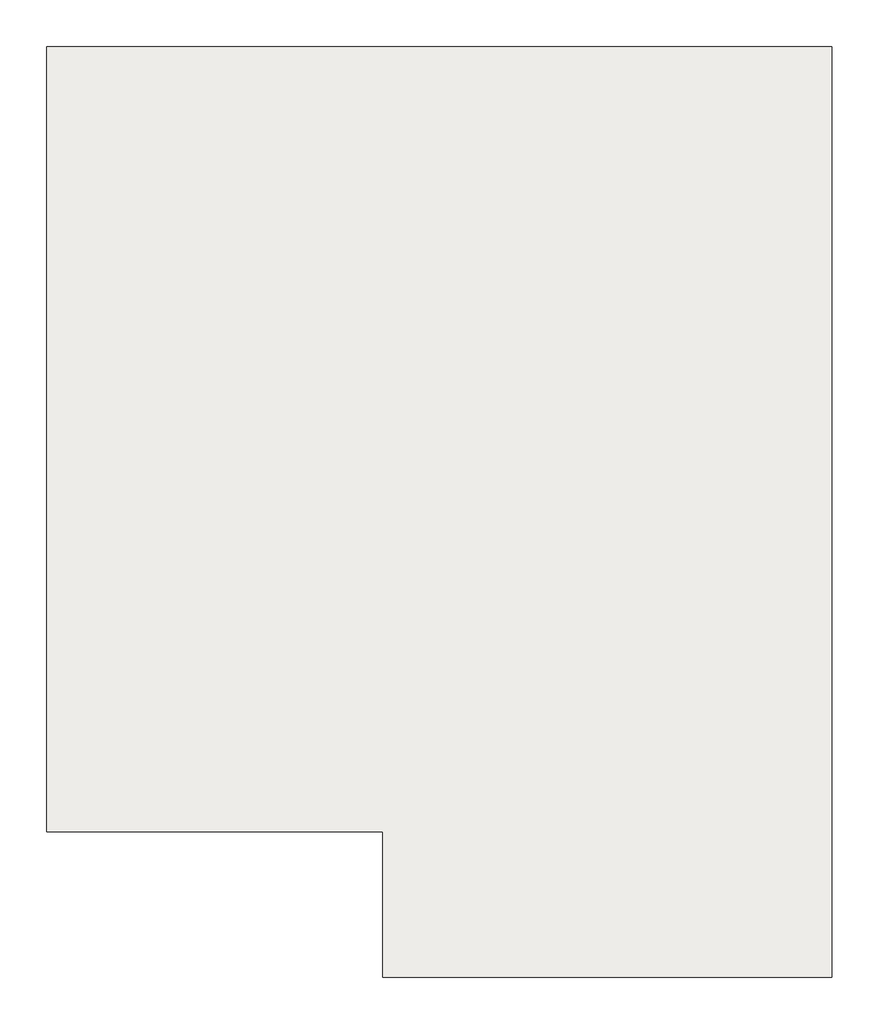
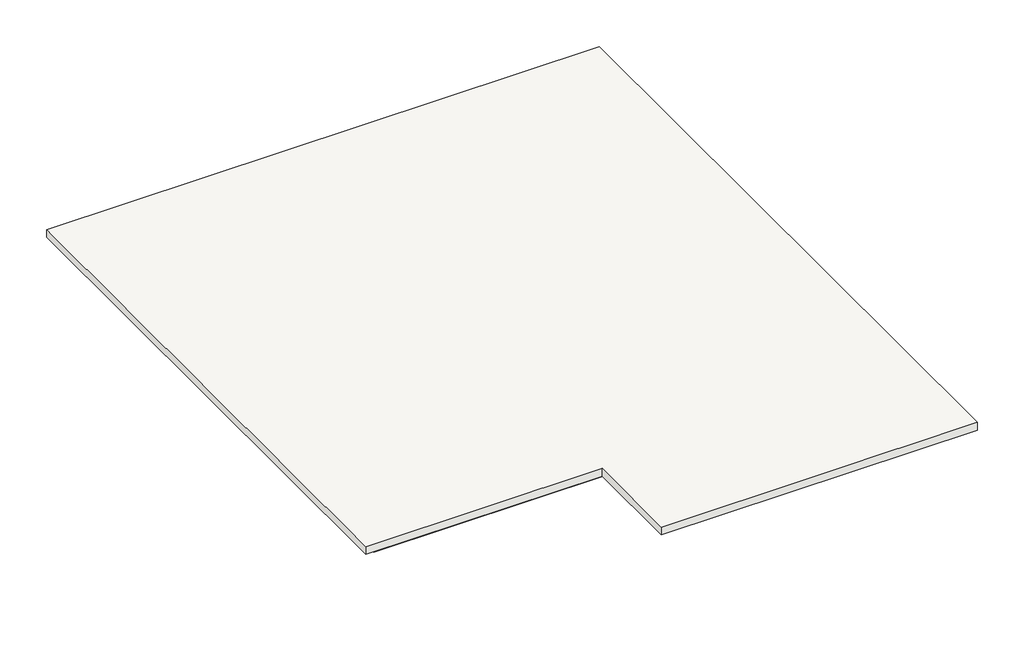
# One storey: 15 beams, 1 slab.
"""IFC4 building model written with IfcOpenShell, lengths in millimetres."""

from ifc_helpers import new_model, si_unit, frame, origin, place, context, project, spatial, polyline, outline, extrude, faceted_brep, element, save

model = new_model("IFC4")

# Units and contexts
model_context = context("Model", 3, world=origin())
ifc_project = project(units=[si_unit("LENGTHUNIT", "METRE", prefix="MILLI")], contexts=[model_context])

# Site, building, storey
site = spatial("IfcSite", under=ifc_project)
building = spatial("IfcBuilding", under=site)
storey = spatial("IfcBuildingStorey", under=building, Name="Çatı Katı", Elevation=100780.0)

# Beams
placement = place(None, origin())
element("IfcBeam", 1, ObjectType="M_Concrete-Rectangular Beam : 300 x 600mm", at=placement, inside=storey, context=model_context, shape_type="SweptSolid", body=[
    extrude(outline(polyline([(-8879.0485128, 8478.2904426), (-8879.0485128, 8778.2904426), (-5329.0485128, 8778.2904426), (-5329.0485128, 8478.2904426), (-8879.0485128, 8478.2904426)])), frame((0.0, 0.0, 100180.0), z_axis=(0.0, 0.0, 1.0), x_axis=(1.0, 0.0, 0.0)), (0.0, 0.0, 1.0), 400.0),
])
element("IfcBeam", 2, ObjectType="M_Concrete-Rectangular Beam : 300 x 600mm", at=placement, inside=storey, context=model_context, shape_type="SweptSolid", body=[
    extrude(outline(polyline([(-2679.0485128, 2578.2904426), (-2979.0485128, 2578.2904426), (-2979.0485128, 4628.2904426), (-2679.0485128, 4628.2904426), (-2679.0485128, 2578.2904426)])), frame((0.0, 0.0, 100180.0), z_axis=(0.0, 0.0, 1.0), x_axis=(1.0, 0.0, 0.0)), (0.0, 0.0, 1.0), 400.0),
])
element("IfcBeam", 3, ObjectType="M_Concrete-Rectangular Beam : 450 x 600mm", at=placement, inside=storey, context=model_context, shape_type="SweptSolid", body=[
    extrude(outline(polyline([(-8954.0485128, -3259.0095568), (-9404.0485128, -3259.0095568), (-9404.0485128, 1978.2904426), (-8954.0485128, 1978.2904426), (-8954.0485128, -3259.0095568)])), frame((0.0, 0.0, 100180.0), z_axis=(0.0, 0.0, 1.0), x_axis=(1.0, 0.0, 0.0)), (0.0, 0.0, 1.0), 400.0),
])
element("IfcBeam", 4, ObjectType="M_Concrete-Rectangular Beam : 450 x 600mm", at=placement, inside=storey, context=model_context, shape_type="SweptSolid", body=[
    extrude(outline(polyline([(-9404.0485128, 8315.590442), (-8954.0485128, 8315.590442), (-8954.0485128, 2578.2904426), (-9404.0485128, 2578.2904426), (-9404.0485128, 8315.590442)])), frame((0.0, 0.0, 100180.0), z_axis=(0.0, 0.0, 1.0), x_axis=(1.0, 0.0, 0.0)), (0.0, 0.0, 1.0), 400.0),
])
element("IfcBeam", 5, ObjectType="M_Concrete-Rectangular Beam : 450 x 600mm", at=placement, inside=storey, context=model_context, shape_type="SweptSolid", body=[
    extrude(outline(polyline([(-14716.3485122, 2053.2904426), (-14716.3485122, 2503.2904426), (-9404.0485128, 2503.2904426), (-9404.0485128, 2053.2904426), (-14716.3485122, 2053.2904426)])), frame((0.0, 0.0, 100180.0), z_axis=(0.0, 0.0, 1.0), x_axis=(1.0, 0.0, 0.0)), (0.0, 0.0, 1.0), 400.0),
])
element("IfcBeam", 6, ObjectType="M_Concrete-Rectangular Beam : 450 x 600mm", at=placement, inside=storey, context=model_context, shape_type="SweptSolid", body=[
    extrude(outline(polyline([(-3141.7485135, 2503.2904426), (-3141.7485135, 2053.2904426), (-8954.0485128, 2053.2904426), (-8954.0485128, 2503.2904426), (-3141.7485135, 2503.2904426)])), frame((0.0, 0.0, 100180.0), z_axis=(0.0, 0.0, 1.0), x_axis=(1.0, 0.0, 0.0)), (0.0, 0.0, 1.0), 400.0),
])
element("IfcBeam", 7, ObjectType="M_Concrete-Rectangular Beam : 450 x 600mm", at=placement, inside=storey, context=model_context, shape_type="SweptSolid", body=[
    extrude(outline(polyline([(-9491.7485135, 8803.2904426), (-9491.7485135, 8353.2904426), (-14729.0485128, 8353.2904426), (-14729.0485128, 8778.2904426), (-15179.0485128, 8778.2904426), (-15179.0485128, 8353.2904426), (-15204.0485128, 8353.2904426), (-15204.0485128, 8803.2904426), (-9491.7485135, 8803.2904426)])), frame((0.0, 0.0, 100180.0), z_axis=(0.0, 0.0, 1.0), x_axis=(1.0, 0.0, 0.0)), (0.0, 0.0, 1.0), 400.0),
])
element("IfcBeam", 8, ObjectType="M_Concrete-Rectangular Beam : 450 x 600mm", at=placement, inside=storey, context=model_context, shape_type="Brep", body=[
    faceted_brep([(-2654.0485128, 1965.590442, 100180.0), (-3104.0485128, 1965.590442, 100180.0), (-3104.0485128, 1965.590442, 100580.0), (-2654.0485128, 1965.590442, 100580.0), (-2654.0485128, -3746.7095574, 100180.0), (-2654.0485128, -3746.7095574, 100580.0), (-2679.0485128, -3746.7095574, 100180.0), (-3104.0485128, -3746.7095574, 100180.0), (-3104.0485128, -3721.7095574, 100180.0), (-2679.0485128, -3721.7095574, 100180.0), (-2679.0485128, -3121.7095574, 100180.0), (-3104.0485128, -3121.7095574, 100180.0), (-3104.0485128, -3746.7095574, 100580.0), (-3104.0485128, -3721.7095574, 100580.0), (-2679.0485128, -3121.7095574, 100580.0), (-3104.0485128, -3121.7095574, 100580.0), (-2679.0485128, -3721.7095574, 100580.0), (-2679.0485128, -3746.7095574, 100580.0)], [[[0, 1, 2, 3]], [[4, 0, 3, 5]], [[1, 0, 4, 6, 7, 8, 9, 10, 11]], [[8, 7, 12, 13]], [[11, 10, 14, 15]], [[10, 9, 16, 14]], [[3, 2, 15, 14, 16, 13, 12, 17, 5]], [[7, 6, 4, 5, 17, 12]], [[9, 8, 13, 16]], [[1, 11, 15, 2]]]),
])
element("IfcBeam", 9, ObjectType="M_Concrete-Rectangular Beam : 450 x 600mm", at=placement, inside=storey, context=model_context, shape_type="SweptSolid", body=[
    extrude(outline(polyline([(-9491.7485135, -3296.7095574), (-9491.7485135, -3746.7095574), (-15204.0485128, -3746.7095574), (-15204.0485128, -3296.7095574), (-15179.0485128, -3296.7095574), (-15179.0485128, -3721.7095574), (-14729.0485128, -3721.7095574), (-14729.0485128, -3296.7095574), (-9491.7485135, -3296.7095574)])), frame((0.0, 0.0, 100180.0), z_axis=(0.0, 0.0, 1.0), x_axis=(1.0, 0.0, 0.0)), (0.0, 0.0, 1.0), 400.0),
])
element("IfcBeam", 10, ObjectType="M_Concrete-Rectangular Beam : 450 x 600mm", at=placement, inside=storey, context=model_context, shape_type="Brep", body=[
    faceted_brep([(-9404.0485128, -3746.7095574, 100180.0), (-8954.0485128, -3746.7095574, 100180.0), (-3129.0485128, -3746.7095574, 100180.0), (-3104.0485128, -3746.7095574, 100180.0), (-3104.0485128, -3746.7095574, 100580.0), (-3129.0485128, -3746.7095574, 100580.0), (-8954.0485128, -3746.7095574, 100580.0), (-9404.0485128, -3746.7095574, 100580.0), (-3129.0485128, -3296.7095574, 100180.0), (-3129.0485128, -3721.7095574, 100180.0), (-3104.0485128, -3721.7095574, 100180.0), (-9404.0485128, -3721.7095574, 100180.0), (-8879.0485128, -3721.7095574, 100180.0), (-8879.0485128, -3296.7095574, 100180.0), (-8879.0485128, -3296.7095574, 100580.0), (-3129.0485128, -3296.7095574, 100580.0), (-3104.0485128, -3721.7095574, 100580.0), (-9404.0485128, -3721.7095574, 100580.0), (-8879.0485128, -3721.7095574, 100580.0), (-3129.0485128, -3721.7095574, 100580.0)], [[[0, 1, 2, 3, 4, 5, 6, 7]], [[8, 9, 10, 3, 2, 1, 0, 11, 12, 13]], [[8, 13, 14, 15]], [[3, 10, 16, 4]], [[12, 11, 17, 18]], [[13, 12, 18, 14]], [[9, 8, 15, 19]], [[10, 9, 19, 16]], [[7, 6, 5, 4, 16, 19, 15, 14, 18, 17]], [[11, 0, 7, 17]]]),
])
element("IfcBeam", 11, ObjectType="M_Concrete-Rectangular Beam : 450 x 600mm", at=placement, inside=storey, context=model_context, shape_type="SweptSolid", body=[
    extrude(outline(polyline([(-14754.0485128, 2590.9904432), (-15204.0485128, 2590.9904432), (-15204.0485128, 8353.2904426), (-15179.0485128, 8353.2904426), (-15179.0485128, 8178.2904426), (-14754.0485128, 8178.2904426), (-14754.0485128, 2590.9904432)])), frame((0.0, 0.0, 100180.0), z_axis=(0.0, 0.0, 1.0), x_axis=(1.0, 0.0, 0.0)), (0.0, 0.0, 1.0), 400.0),
])
element("IfcBeam", 12, ObjectType="M_Concrete-Rectangular Beam : 450 x 600mm", at=placement, inside=storey, context=model_context, shape_type="SweptSolid", body=[
    extrude(outline(polyline([(-15204.0485128, 1965.590442), (-14754.0485128, 1965.590442), (-14754.0485128, -3121.7095574), (-15179.0485128, -3121.7095574), (-15179.0485128, -3296.7095574), (-15204.0485128, -3296.7095574), (-15204.0485128, 1965.590442)])), frame((0.0, 0.0, 100180.0), z_axis=(0.0, 0.0, 1.0), x_axis=(1.0, 0.0, 0.0)), (0.0, 0.0, 1.0), 400.0),
])
element("IfcBeam", 13, ObjectType="M_Concrete-Rectangular Beam : 450 x 600mm", at=placement, inside=storey, context=model_context, shape_type="SweptSolid", body=[
    extrude(outline(polyline([(-8954.0485128, -5771.7095574), (-9404.0485128, -5771.7095574), (-9404.0485128, -3746.7095574), (-8954.0485128, -3746.7095574), (-8954.0485128, -5771.7095574)])), frame((0.0, 0.0, 100180.0), z_axis=(0.0, 0.0, 1.0), x_axis=(1.0, 0.0, 0.0)), (0.0, 0.0, 1.0), 400.0),
])
element("IfcBeam", 14, ObjectType="M_Concrete-Rectangular Beam : 450 x 600mm", at=placement, inside=storey, context=model_context, shape_type="Brep", body=[
    faceted_brep([(-3129.0485128, -3746.7095574, 100180.0), (-3129.0485128, -5771.7095574, 100180.0), (-3129.0485128, -5771.7095574, 100580.0), (-3129.0485128, -3746.7095574, 100580.0), (-2679.0485128, -5771.7095574, 100180.0), (-3104.0485128, -3746.7095574, 100180.0), (-2679.0485128, -3746.7095574, 100180.0), (-2679.0485128, -3746.7095574, 100580.0), (-2679.0485128, -5771.7095574, 100580.0), (-3104.0485128, -3746.7095574, 100580.0)], [[[0, 1, 2, 3]], [[4, 1, 0, 5, 6]], [[4, 6, 7, 8]], [[1, 4, 8, 2]], [[6, 5, 0, 3, 9, 7]], [[3, 2, 8, 7, 9]]]),
])
element("IfcBeam", 15, ObjectType="M_Concrete-Rectangular Beam : 450 x 600mm", at=placement, inside=storey, context=model_context, shape_type="SweptSolid", body=[
    extrude(outline(polyline([(-8954.0485128, -6221.7095574), (-8954.0485128, -5771.7095574), (-3129.0485128, -5771.7095574), (-3129.0485128, -6221.7095574), (-8954.0485128, -6221.7095574)])), frame((0.0, 0.0, 100180.0), z_axis=(0.0, 0.0, 1.0), x_axis=(1.0, 0.0, 0.0)), (0.0, 0.0, 1.0), 400.0),
])

# Slab
element("IfcSlab", 16, ObjectType="Generic 200mm", at=placement, inside=storey, context=model_context, shape_type="SweptSolid", body=[
    extrude(outline(polyline([(-2179.0485128, 9278.2904426), (-2179.0485128, -6721.7095574), (-9904.0485128, -6721.7095574), (-9904.0485128, -4221.7095574), (-15679.0485128, -4221.7095574), (-15679.0485128, 9278.2904426), (-2179.0485128, 9278.2904426)])), frame((0.0, 0.0, 100580.0), z_axis=(0.0, 0.0, 1.0), x_axis=(1.0, 0.0, 0.0)), (0.0, 0.0, 1.0), 200.0),
])

save(model, "model.ifc")

# Revit data of these elements
# Type "M_Concrete-Rectangular Beam : 300 x 600mm"
#   Length [instance default] = 152.4 cm
#   b = 30 cm
#   h = 60 cm
#   Structural Material [instance default] = Concrete, Cast-in-Place gray
#   Assembly Code = ""
# Type "M_Concrete-Rectangular Beam : 450 x 600mm"
#   Length [instance default] = 152.4 cm
#   b = 45 cm
#   h = 60 cm
#   Structural Material [instance default] = Concrete, Cast-in-Place gray
#   Assembly Code = ""
# Type "Generic 200mm"
#   Function = 0
#   Layers, outside or top first: 20 cm "Concrete, Cast-in-Place gray" (function 1)
# Elements 1, 2 (IfcBeam, "M_Concrete-Rectangular Beam : 300 x 600mm")
#   Comments = ""
#   Structural Material = Concrete, Cast-in-Place gray
#   Phase Created = New Construction
#   Materials on its faces: "Concrete, Cast-in-Place gray"
# Elements 3, 4, 5, 6, 7, 8, 9, 10, 11, 12 (IfcBeam, "M_Concrete-Rectangular Beam : 450 x 600mm")
#   Comments = ""
#   Structural Material = Concrete, Cast-in-Place gray
#   Phase Created = New Construction
#   Materials on its faces: "Concrete, Cast-in-Place gray"
# Elements 13, 14, 15 (IfcBeam, "M_Concrete-Rectangular Beam : 450 x 600mm")
#   Structural Material = Concrete, Cast-in-Place gray
#   Phase Created = New Construction
#   Materials on its faces: "Concrete, Cast-in-Place gray"
# Element 16 (IfcSlab, "Generic 200mm")
#   Height Offset From Level = 0 cm
#   built-in parameter 1001954 = 1
#   Phase Created = New Construction
#   Materials on its faces: "Concrete, Cast-in-Place gray"
# Materials
#   "Concrete, Cast-in-Place gray": class "Concrete", colour RGB 192 192 192, transparency 0, Description = "Cast-in-place concrete", Cost = 0
